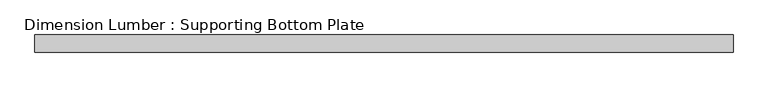
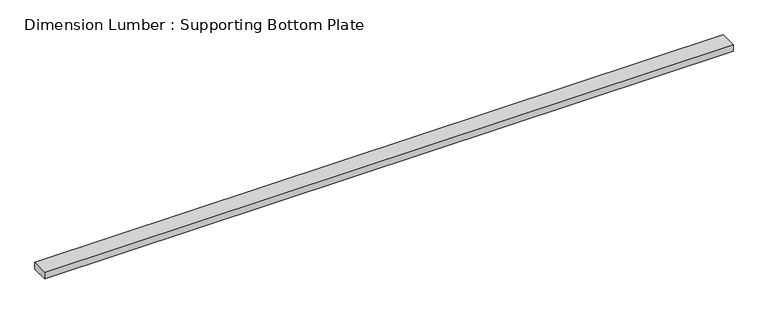
"""IFC4 building model written with IfcOpenShell, lengths in millimetres: beam geometry, Dimension Lumber : Supporting Bottom Plate."""

from ifc_helpers import new_model, si_unit, frame, origin, place, context, project, spatial, polyline, outline, extrude, source, transform, mapped, element, save


def dimension_lumber_supporting_bottom_plate_2403c2db(model_context):
    return source(origin(), model_context, "Body", "SweptSolid", [
        extrude(outline(polyline([(1858.9625, 44.45), (1858.9625, -44.45), (-1770.0625, -44.45), (-1770.0625, 44.45), (1858.9625, 44.45)])), frame((0.0, 0.0, -19.05), z_axis=(0.0, 0.0, 1.0), x_axis=(1.0, 0.0, 0.0)), (0.0, 0.0, 1.0), 38.1),
    ])


if __name__ == "__main__":
    model = new_model("IFC4")
    model_context = context("Model", 3, world=origin())
    ifc_project = project(units=[si_unit("LENGTHUNIT", "METRE", prefix="MILLI")], contexts=[model_context])
    site = spatial("IfcSite", under=ifc_project)
    building = spatial("IfcBuilding", under=site)
    placement = place(None, origin())
    dimension_lumber_supporting_bottom_plate_shape = dimension_lumber_supporting_bottom_plate_2403c2db(model_context)
    element("IfcBeam", 1, ObjectType="Dimension Lumber : Supporting Bottom Plate", at=placement, inside=building, context=model_context, shape_type="MappedRepresentation", body=[
        mapped(dimension_lumber_supporting_bottom_plate_shape, transform((0.0, 0.0, 0.0), x_axis=(1.0, 0.0, 0.0), y_axis=(0.0, 1.0, 0.0), z_axis=(0.0, 0.0, 1.0))),
    ])
    save(model, "model.ifc")

# Revit data of these elements
# Type "Dimension Lumber : Supporting Bottom Plate"
#   Assembly Code = "B10"
#   A = 0.0364583 SF
#   Length [instance default] = 5' - 0"
#   b = 0' - 3 1/2"
#   d = 0' - 1 1/2"
#   Structural Material [instance default] = Softwood, Lumber
# Element 1 (IfcBeam, "Dimension Lumber : Supporting Bottom Plate")
#   Structural Material = Douglas Fir #2
#   Materials on its faces: "Douglas Fir #2"
# Materials
#   "Softwood, Lumber": class "Wood", colour RGB 223 192 134, transparency 0, Description = "Pinus Echinata", Cost = 0
#   "Douglas Fir #2": class "Wood", colour RGB 223 192 134, transparency 0, Description = "Pinus Echinata", Cost = 0
